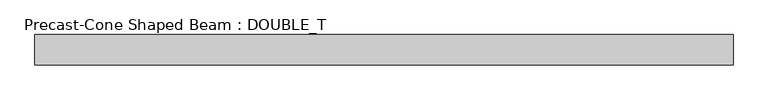
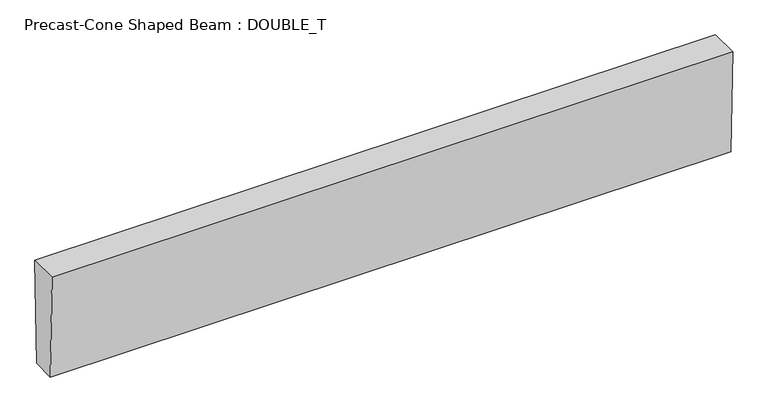
"""IFC4 building model written with IfcOpenShell, lengths in millimetres: beam geometry, Precast-Cone Shaped Beam : DOUBLE_T."""

from ifc_helpers import new_model, si_unit, frame, origin, place, context, project, spatial, polyline, outline, extrude, source, transform, mapped, element, save


def precast_cone_shaped_beam_double_t_8ba99103(model_context):
    return source(origin(), model_context, "Body", "SweptSolid", [
        extrude(outline(polyline([(50.8, -228.6), (-50.8, -228.6), (-63.5, 228.6), (63.5, 228.6), (50.8, -228.6)])), frame((-1610.51875, 0.0, 0.0), z_axis=(1.0, 0.0, 0.0), x_axis=(0.0, 1.0, 0.0)), (0.0, 0.0, 1.0), 2908.3),
    ])


if __name__ == "__main__":
    model = new_model("IFC4")
    model_context = context("Model", 3, world=origin())
    ifc_project = project(units=[si_unit("LENGTHUNIT", "METRE", prefix="MILLI")], contexts=[model_context])
    site = spatial("IfcSite", under=ifc_project)
    building = spatial("IfcBuilding", under=site)
    placement = place(None, origin())
    precast_cone_shaped_beam_double_t_shape = precast_cone_shaped_beam_double_t_8ba99103(model_context)
    element("IfcBeam", 1, ObjectType="Precast-Cone Shaped Beam : DOUBLE_T", at=placement, inside=building, context=model_context, shape_type="MappedRepresentation", body=[
        mapped(precast_cone_shaped_beam_double_t_shape, transform((0.0, 0.0, 0.0), x_axis=(1.0, 0.0, 0.0), y_axis=(0.0, 1.0, 0.0), z_axis=(0.0, 0.0, 1.0))),
    ])
    save(model, "model.ifc")

# Revit data of these elements
# Type "Precast-Cone Shaped Beam : DOUBLE_T"
#   Top Width = 0' - 5"
#   Tie Rod Weight [instance default] = 30
#   Tie Rod W [instance default] = 0.0660938 kip
#   Single Rebar Weight [instance default] = 50
#   Single Rebar W [instance default] = 0.110156 kip
#   Rebar Grids Weight [instance default] = 100
#   Rebar Grids W [instance default] = 0.220313 kip
#   Depth = 1' - 6"
#   Bottom Width = 0' - 4"
#   Length [instance default] = 5' - 0"
#   Structural Material [instance default] = Concrete, Precast
#   Assembly Code = ""
# Element 1 (IfcBeam, "Precast-Cone Shaped Beam : DOUBLE_T")
#   Length = 9' - 7 3/16"
#   Structural Material = Concrete - Precast Concrete - Normal Weight Concrete - 5 ksi
#   Materials on its faces: "Concrete - Precast Concrete - Normal Weight Concrete - 5 ksi"
# Materials
#   "Concrete, Precast": class "Concrete", colour RGB 198 187 187, transparency 0, Description = "Precast concrete", Cost = 0
#   "Concrete - Precast Concrete - Normal Weight Concrete - 5 ksi": class "Concrete", colour RGB 198 187 187, transparency 0, Cost = 0
